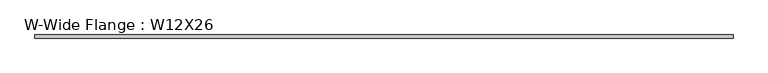
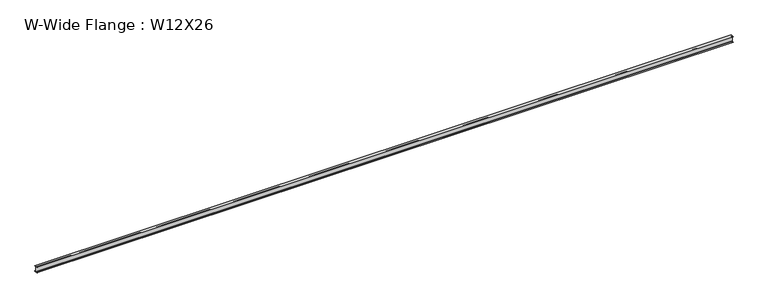
"""IFC4 building model written with IfcOpenShell, lengths in millimetres: beam geometry, W-Wide Flange : W12X26."""

from ifc_helpers import new_model, si_unit, point, frame, frame_2d, origin, place, context, project, spatial, polyline, circle_curve, trimmed, segment, composite_curve, outline, extrude, source, transform, mapped, element, save


def w_wide_flange_w12x26_8bffb349(model_context):
    return source(origin(), model_context, "Body", "SweptSolid", [
        extrude(outline(composite_curve([segment(polyline([(82.4011719, -145.5539063), (82.4011719, -155.178125), (-82.4011719, -155.178125), (-82.4011719, -145.5539063), (-20.2902344, -145.5539063)]), True, "CONTINUOUS"), segment(trimmed(circle_curve(frame_2d((-20.2902344, -128.190625)), 17.3632812), [point((-20.2902344, -145.5539063))], [point((-2.9269531, -128.190625))], True, "CARTESIAN"), True, "CONTINUOUS"), segment(polyline([(-2.9269531, -128.190625), (-2.9269531, 128.190625)]), True, "CONTINUOUS"), segment(trimmed(circle_curve(frame_2d((-20.2902344, 128.190625)), 17.3632812), [point((-2.9269531, 128.190625))], [point((-20.2902344, 145.5539062))], True, "CARTESIAN"), True, "CONTINUOUS"), segment(polyline([(-20.2902344, 145.5539062), (-82.4011719, 145.5539062), (-82.4011719, 155.178125), (82.4011719, 155.178125), (82.4011719, 145.5539062), (20.2902344, 145.5539062)]), True, "CONTINUOUS"), segment(trimmed(circle_curve(frame_2d((20.2902344, 128.190625)), 17.3632812), [point((20.2902344, 145.5539062))], [point((2.9269531, 128.190625))], True, "CARTESIAN"), True, "CONTINUOUS"), segment(polyline([(2.9269531, 128.190625), (2.9269531, -128.190625)]), True, "CONTINUOUS"), segment(trimmed(circle_curve(frame_2d((20.2902344, -128.190625)), 17.3632812), [point((2.9269531, -128.190625))], [point((20.2902344, -145.5539063))], True, "CARTESIAN"), True, "CONTINUOUS"), segment(polyline([(20.2902344, -145.5539063), (82.4011719, -145.5539063)]), True, "CONTINUOUS")], self_intersect=False)), frame((-18168.1309128, 0.0, 0.0), z_axis=(1.0, 0.0, 0.0), x_axis=(0.0, 1.0, 0.0)), (0.0, 0.0, 1.0), 36321.8254975),
    ])


if __name__ == "__main__":
    model = new_model("IFC4")
    model_context = context("Model", 3, world=origin())
    ifc_project = project(units=[si_unit("LENGTHUNIT", "METRE", prefix="MILLI")], contexts=[model_context])
    site = spatial("IfcSite", under=ifc_project)
    building = spatial("IfcBuilding", under=site)
    placement = place(None, origin())
    w_wide_flange_w12x26_shape = w_wide_flange_w12x26_8bffb349(model_context)
    element("IfcBeam", 1, ObjectType="W-Wide Flange : W12X26", at=placement, inside=building, context=model_context, shape_type="MappedRepresentation", body=[
        mapped(w_wide_flange_w12x26_shape, transform((0.0, 0.0, 0.0), x_axis=(1.0, 0.0, 0.0), y_axis=(0.0, 1.0, 0.0), z_axis=(0.0, 0.0, 1.0))),
    ])
    save(model, "model.ifc")

# Revit data of these elements
# Type "W-Wide Flange : W12X26"
#   Assembly Code = "B10"
#   W = 26
#   Length [instance default] = 5' - 0"
#   bf = 0' - 6 125/256"
#   d = 1' - 0 7/32"
#   k = 0' - 1 1/16"
#   k2 = 0' - 0 175/256"
#   tf = 0' - 0 97/256"
#   tw = 0' - 0 59/256"
#   A = 0.053125 SF
#   Structural Material [instance default] = none
# Element 1 (IfcBeam, "W-Wide Flange : W12X26")
#   Structural Material = Dark metal
#   Materials on its faces: "Dark metal"
# Materials
#   "Dark metal": class "Generic", colour RGB 44 29 29, transparency 0, Cost = 0
